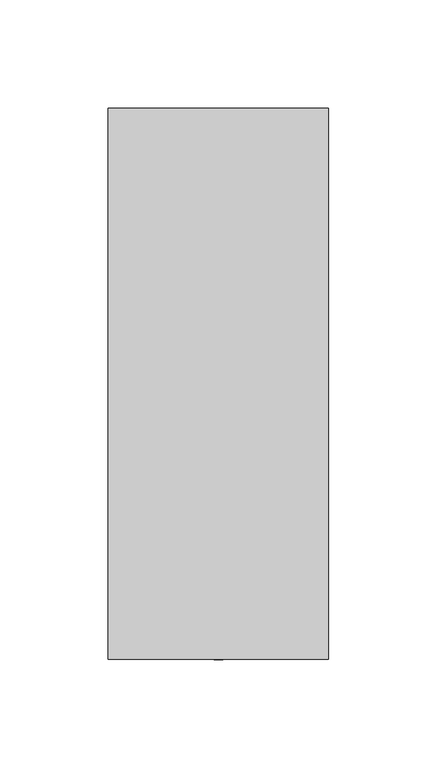
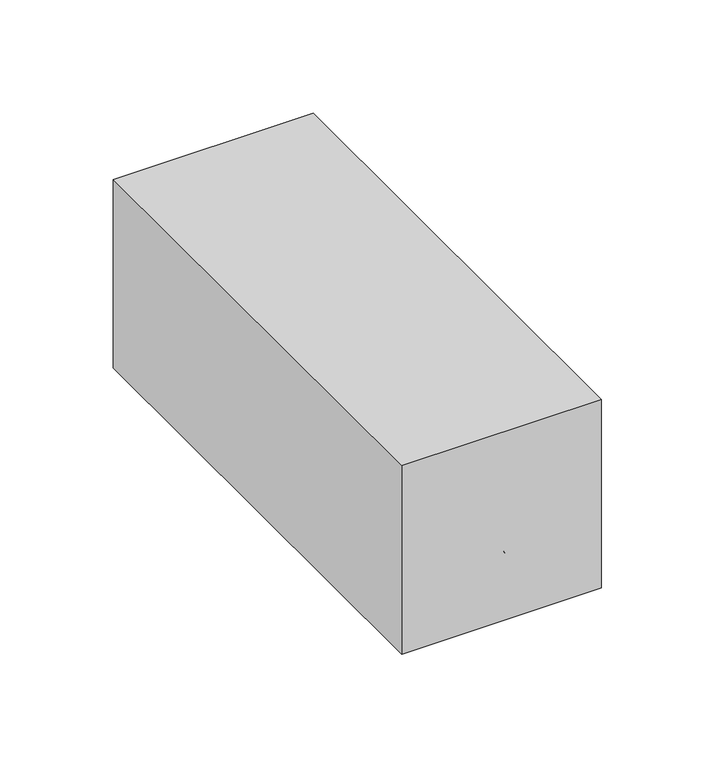
"""IFC4 building model written with IfcOpenShell, lengths in millimetres: proxy geometry, M0750 - Flowmeter, Air, Connect W50 PSI Supply : M0750 - Flowmeter, Air, Connect W50 PSI Supply."""

import ifcopenshell
import ifcopenshell.guid

model = None  # the IFC model being written
_history = None  # IfcOwnerHistory: only IFC2X3 demands one
_inside = {}  # id of a spatial element -> (the spatial element, [elements in it])
_under = {}  # id of a project, library or spatial element -> (it, [spatial elements below it])
_declared = {}  # id of a project -> (the project, [libraries it declares])
_typed = {}  # id of a type object -> (the type object, [elements of that type])
_made_of = {}  # id of a material, layer set ... -> (it, [elements and type objects made of it])


def new_model(schema):
    """Start an empty IFC model of exactly this schema.

    Asked for "IFC4X3", IfcOpenShell would pick the latest addendum, in which some entities
    have other attributes; the version numbers below select the first issue.
    IFC2X3 requires an IfcOwnerHistory on every rooted entity: one is made here for all.
    """
    global model, _history
    if schema == "IFC4X3":
        model = ifcopenshell.file(schema_version=(4, 3, 0, 0))
    else:
        model = ifcopenshell.file(schema=schema)
    _inside.clear()
    _under.clear()
    _declared.clear()
    _typed.clear()
    _made_of.clear()
    _history = None
    if model.schema == "IFC2X3":
        org = make("IfcOrganization", Name="unknown")
        user = make(
            "IfcPersonAndOrganization",
            ThePerson=make("IfcPerson", FamilyName="unknown"),
            TheOrganization=org,
        )
        app = make(
            "IfcApplication",
            ApplicationDeveloper=org,
            Version="unknown",
            ApplicationFullName="unknown",
            ApplicationIdentifier="unknown",
        )
        _history = make(
            "IfcOwnerHistory",
            OwningUser=user,
            OwningApplication=app,
            ChangeAction="ADDED",
            CreationDate=0,
        )
    return model


def make(cls, **values):
    """One entity of the class cls with the attributes given. An attribute that is None is left unset."""
    return model.create_entity(
        cls, **{name: value for name, value in values.items() if value is not None}
    )


def rooted(cls, **values):
    """An entity with a GlobalId (a new one), such as an element, a storey or a relation."""
    return make(cls, GlobalId=ifcopenshell.guid.new(), OwnerHistory=_history, **values)


def si_unit(unit_type, name, prefix=None):
    """IfcSIUnit, for example si_unit("LENGTHUNIT", "METRE", prefix="MILLI")."""
    return make("IfcSIUnit", UnitType=unit_type, Prefix=prefix, Name=name)


def assignment(units):
    """IfcUnitAssignment: the units of a project."""
    return None if units is None else make("IfcUnitAssignment", Units=units)


def point(xyz):
    """IfcCartesianPoint."""
    return None if xyz is None else make("IfcCartesianPoint", Coordinates=xyz)


def direction(xyz):
    """IfcDirection."""
    return None if xyz is None else make("IfcDirection", DirectionRatios=xyz)


def frame(location, z_axis=None, x_axis=None):
    """IfcAxis2Placement3D, a coordinate frame: its origin and axes. An axis left out is left unset."""
    return make(
        "IfcAxis2Placement3D",
        Location=point(location),
        Axis=direction(z_axis),
        RefDirection=direction(x_axis),
    )


def frame_2d(location, x_axis=None):
    """IfcAxis2Placement2D, a coordinate frame in the plane: its origin and x axis."""
    return make(
        "IfcAxis2Placement2D", Location=point(location), RefDirection=direction(x_axis)
    )


def origin():
    """The frame at (0, 0, 0) with its axes left unset."""
    return frame((0.0, 0.0, 0.0))


def origin_with_axes():
    """The frame at (0, 0, 0) with the z axis (0, 0, 1) and the x axis (1, 0, 0) written out."""
    return frame((0.0, 0.0, 0.0), z_axis=(0.0, 0.0, 1.0), x_axis=(1.0, 0.0, 0.0))


def place(relative_to, where):
    """IfcLocalPlacement: puts the frame where relative to a parent placement (None: the world)."""
    return make(
        "IfcLocalPlacement", PlacementRelTo=relative_to, RelativePlacement=where
    )


def context(
    kind, dimensions, precision=None, world=None, true_north=None, identifier=None
):
    """IfcGeometricRepresentationContext, for example the 3D "Model" context."""
    return make(
        "IfcGeometricRepresentationContext",
        ContextIdentifier=identifier,
        ContextType=kind,
        CoordinateSpaceDimension=dimensions,
        Precision=precision,
        WorldCoordinateSystem=world,
        TrueNorth=true_north,
    )


def project(units=None, contexts=None):
    """IfcProject with its units and contexts."""
    return rooted(
        "IfcProject",
        Name="project",
        RepresentationContexts=contexts,
        UnitsInContext=assignment(units),
    )


def spatial(cls, under=None, at=None, **own):
    """A site, building, storey or space (cls), placed at a placement, below another one or the project."""
    s = rooted(cls, ObjectPlacement=at, **own)
    if under is not None:
        _under.setdefault(under.id(), (under, []))[1].append(s)
    return s


def polyline(points):
    """IfcPolyline through the points."""
    return make("IfcPolyline", Points=[point(p) for p in points])


def circle_curve(where, radius):
    """IfcCircle in the frame where."""
    return make("IfcCircle", Position=where, Radius=radius)


def trimmed(basis, trim1, trim2, sense, master):
    """IfcTrimmedCurve: the piece of a basis curve between two trims."""
    return make(
        "IfcTrimmedCurve",
        BasisCurve=basis,
        Trim1=trim1,
        Trim2=trim2,
        SenseAgreement=sense,
        MasterRepresentation=master,
    )


def segment(curve, same_sense, transition):
    """IfcCompositeCurveSegment."""
    return make(
        "IfcCompositeCurveSegment",
        Transition=transition,
        SameSense=same_sense,
        ParentCurve=curve,
    )


def composite_curve(segments, self_intersect=None):
    """IfcCompositeCurve: segments joined end to end."""
    return make("IfcCompositeCurve", Segments=segments, SelfIntersect=self_intersect)


def outline(outer, holes=None, kind="AREA"):
    """IfcArbitraryClosedProfileDef: a profile drawn as a closed curve; with holes, ...WithVoids."""
    if holes is None:
        return make("IfcArbitraryClosedProfileDef", ProfileType=kind, OuterCurve=outer)
    return make(
        "IfcArbitraryProfileDefWithVoids",
        ProfileType=kind,
        OuterCurve=outer,
        InnerCurves=holes,
    )


def extrude(swept, where, along, depth):
    """IfcExtrudedAreaSolid: the profile swept, set in the frame where, extruded along a direction by depth."""
    return make(
        "IfcExtrudedAreaSolid",
        SweptArea=swept,
        Position=where,
        ExtrudedDirection=direction(along),
        Depth=depth,
    )


def shape(context_of_items, identifier, shape_type, items):
    """IfcShapeRepresentation: the items that make up one representation, for example the "Body"."""
    return make(
        "IfcShapeRepresentation",
        ContextOfItems=context_of_items,
        RepresentationIdentifier=identifier,
        RepresentationType=shape_type,
        Items=items,
    )


def source(mapping_origin, context_of_items, identifier, shape_type, items):
    """IfcRepresentationMap: a shape defined once, which mapped items show again and again."""
    return make(
        "IfcRepresentationMap",
        MappingOrigin=mapping_origin,
        MappedRepresentation=shape(context_of_items, identifier, shape_type, items),
    )


def transform(
    local_origin,
    x_axis=None,
    y_axis=None,
    z_axis=None,
    scale=None,
    scale2=None,
    scale3=None,
    uniform=True,
):
    """IfcCartesianTransformationOperator3D, or its non-uniform kind. x_axis, y_axis, z_axis: its Axis1, 2, 3."""
    if uniform:
        return make(
            "IfcCartesianTransformationOperator3D",
            Axis1=direction(x_axis),
            Axis2=direction(y_axis),
            LocalOrigin=point(local_origin),
            Scale=scale,
            Axis3=direction(z_axis),
        )
    return make(
        "IfcCartesianTransformationOperator3DnonUniform",
        Axis1=direction(x_axis),
        Axis2=direction(y_axis),
        LocalOrigin=point(local_origin),
        Scale=scale,
        Axis3=direction(z_axis),
        Scale2=scale2,
        Scale3=scale3,
    )


def mapped(mapping_source, mapping_target):
    """IfcMappedItem: shows the shape of a source again, moved by a transform."""
    return make(
        "IfcMappedItem", MappingSource=mapping_source, MappingTarget=mapping_target
    )


def made_of(thing, what):
    """Note that an element or type object is made of a material, layer set ...; save() writes the relation."""
    if what is not None:
        _made_of.setdefault(what.id(), (what, []))[1].append(thing)
    return thing


def element(
    cls,
    number,
    at=None,
    inside=None,
    cuts=None,
    type_object=None,
    material=None,
    context=None,
    identifier="Body",
    shape_type=None,
    held_by="IfcProductDefinitionShape",
    body=None,
    shapes=None,
    **own,
):
    """One element of the class cls, such as IfcWall. Its Tag is "e" and its number.

    at: its placement. inside: the storey or other place that contains it. cuts: it is an
    opening in that element (IfcRelVoidsElement). A single representation is given by context,
    identifier, shape_type and body (its items); several are given by shapes. held_by: the class
    of the entity that holds the representations. save() writes the other relations.
    """
    e = rooted(cls, Tag="e%d" % number, ObjectPlacement=at, **own)
    if body is not None:
        shapes = [shape(context, identifier, shape_type, body)]
    if shapes is not None:
        e.Representation = make(held_by, Representations=shapes)
    if inside is not None:
        _inside.setdefault(inside.id(), (inside, []))[1].append(e)
    if cuts is not None:
        rooted(
            "IfcRelVoidsElement", RelatingBuildingElement=cuts, RelatedOpeningElement=e
        )
    if type_object is not None:
        _typed.setdefault(type_object.id(), (type_object, []))[1].append(e)
    return made_of(e, material)


def aggregate(whole, parts):
    """IfcRelAggregates: a whole, such as a stair, and the parts it consists of."""
    return rooted("IfcRelAggregates", RelatingObject=whole, RelatedObjects=parts)


def save(model, path):
    """Write the relations noted so far, then the file.

    IfcRelAggregates (storeys below a building ...), IfcRelContainedInSpatialStructure (elements
    in a storey), IfcRelDefinesByType, IfcRelAssociatesMaterial and IfcRelDeclares: one each for
    every whole, place, type object, material and project.
    """
    for whole, parts in _under.values():
        aggregate(whole, parts)
    for where, things in _inside.values():
        rooted(
            "IfcRelContainedInSpatialStructure",
            RelatedElements=things,
            RelatingStructure=where,
        )
    for kind, things in _typed.values():
        rooted("IfcRelDefinesByType", RelatedObjects=things, RelatingType=kind)
    for what, things in _made_of.values():
        rooted("IfcRelAssociatesMaterial", RelatedObjects=things, RelatingMaterial=what)
    for by, libraries in _declared.values():
        rooted("IfcRelDeclares", RelatingContext=by, RelatedDefinitions=libraries)
    model.write(path)


def plane_surface(at):
    """IfcPlane: the flat surface through the origin of the frame at, square to its z axis."""
    return make("IfcPlane", Position=at)


def cylinder_surface(at, radius):
    """IfcCylindricalSurface: all points at the distance radius from the z axis of the frame at."""
    return make("IfcCylindricalSurface", Position=at, Radius=radius)


def revolved_surface(curve, axis_point, axis_direction):
    """IfcSurfaceOfRevolution: the curve turned about the line through axis_point along axis_direction."""
    return make(
        "IfcSurfaceOfRevolution",
        SweptCurve=make("IfcArbitraryOpenProfileDef", ProfileType="CURVE", Curve=curve),
        AxisPosition=make("IfcAxis1Placement", Location=point(axis_point), Axis=direction(axis_direction)),
    )


def advanced_brep(points, edges, surfaces, faces):
    """IfcAdvancedBrep: a solid bounded by faces that lie on surfaces and meet in shared edges.

    An edge is (start, end): straight between two places in points (the first is 0);
    or (start, end, curve); or (start, end, curve, False) where it runs against its curve.
    A face is (place in surfaces, loops), or (place, loops, False) where it looks against
    its surface's normal. A loop lists edges by number (the first is 1), with a minus sign
    where the edge is run from its end to its start. The first loop is the outer one.
    """
    corners = [point(p) for p in points]
    vertices = [make("IfcVertexPoint", VertexGeometry=c) for c in corners]
    made = []
    for start, end, *more in edges:
        made.append(
            make(
                "IfcEdgeCurve",
                EdgeStart=vertices[start],
                EdgeEnd=vertices[end],
                EdgeGeometry=more[0] if more else make("IfcPolyline", Points=[corners[start], corners[end]]),
                SameSense=more[1] if len(more) > 1 else True,
            )
        )
    hull = []
    for where, loops, *sense in faces:
        bounds = []
        for j, loop in enumerate(loops):
            ring = [make("IfcOrientedEdge", EdgeElement=made[abs(k) - 1], Orientation=k > 0) for k in loop]
            bounds.append(
                make(
                    "IfcFaceOuterBound" if j == 0 else "IfcFaceBound",
                    Bound=make("IfcEdgeLoop", EdgeList=ring),
                    Orientation=True,
                )
            )
        hull.append(make("IfcAdvancedFace", Bounds=bounds, FaceSurface=surfaces[where], SameSense=sense[0] if sense else True))
    return make("IfcAdvancedBrep", Outer=make("IfcClosedShell", CfsFaces=hull))


def specialty_equipment_235a6406(model_context):
    return source(origin(), model_context, "Body", "SolidModel", [
        extrude(outline(polyline([(-50.8, 254.0), (50.8, 254.0), (50.8, 0.0), (-50.8, 0.0), (-50.8, 254.0)])), origin_with_axes(), (0.0, 0.0, 1.0), 101.6),
        extrude(outline(composite_curve([segment(trimmed(circle_curve(frame_2d((0.0, 43.7511243)), 11.1125), [point((-11.1125, 43.7511243))], [point((11.1125, 43.7511243))], False, "CARTESIAN"), True, "CONTINUOUS"), segment(trimmed(circle_curve(frame_2d((0.0, 43.7511243)), 11.1125), [point((11.1125, 43.7511243))], [point((-11.1125, 43.7511243))], False, "CARTESIAN"), True, "CONTINUOUS")], self_intersect=False)), origin_with_axes(), (0.0, 0.0, 1.0), 12.1432676),
        extrude(outline(composite_curve([segment(trimmed(circle_curve(frame_2d((0.0, 43.7511243)), 6.35), [point((-6.35, 43.7511243))], [point((6.35, 43.7511243))], False, "CARTESIAN"), True, "CONTINUOUS"), segment(trimmed(circle_curve(frame_2d((0.0, 43.7511243)), 6.35), [point((6.35, 43.7511243))], [point((-6.35, 43.7511243))], False, "CARTESIAN"), True, "CONTINUOUS")], self_intersect=False)), frame((0.0, 0.0, 12.1432676), z_axis=(0.0, 0.0, 1.0), x_axis=(1.0, 0.0, 0.0)), (0.0, 0.0, 1.0), 11.6740858),
        extrude(outline(composite_curve([segment(trimmed(circle_curve(frame_2d((0.0, 43.7511243)), 11.1125), [point((-11.1125, 43.7511243))], [point((11.1125, 43.7511243))], False, "CARTESIAN"), True, "CONTINUOUS"), segment(trimmed(circle_curve(frame_2d((0.0, 43.7511243)), 11.1125), [point((11.1125, 43.7511243))], [point((-11.1125, 43.7511243))], False, "CARTESIAN"), True, "CONTINUOUS")], self_intersect=False)), frame((0.0, 0.0, 12.8429111), z_axis=(0.0, 0.0, 1.0), x_axis=(1.0, 0.0, 0.0)), (0.0, 0.0, 1.0), 3.7345018),
        advanced_brep(
        [(0.0, 195.0035492, 41.6430751), (0.0, 195.0035492, 28.9430751), (0.0, 77.2962509, 43.2305751), (0.0, 77.2962509, 27.3555751)],
        [
            (0, 1, circle_curve(frame((0.0, 195.0035492, 35.2930751), z_axis=(0.0, 1.0, 0.0), x_axis=(0.0, 0.0, 1.0)), 6.35)),
            (1, 0, circle_curve(frame((0.0, 195.0035492, 35.2930751), z_axis=(0.0, 1.0, 0.0), x_axis=(0.0, 0.0, -1.0)), 6.35)),
            (2, 3, circle_curve(frame((0.0, 77.2962509, 35.2930751), z_axis=(0.0, -1.0, 0.0), x_axis=(0.0, 0.0, -1.0)), 7.9375)),
            (3, 2, circle_curve(frame((0.0, 77.2962509, 35.2930751), z_axis=(0.0, -1.0, 0.0), x_axis=(0.0, 0.0, 1.0)), 7.9375)),
            (3, 1),
            (0, 2),
        ],
        [
            plane_surface(frame((0.0, 195.0035492, 35.2930751), z_axis=(0.0, 1.0, 0.0), x_axis=(1.0, 0.0, 0.0))),
            plane_surface(frame((0.0, 77.2962509, 35.2930751), z_axis=(0.0, -1.0, 0.0), x_axis=(1.0, 0.0, 0.0))),
            revolved_surface(polyline([(0.0, 195.0035492, 41.64307510053948), (0.0, 77.29625090000002, 43.2305751)]), (0.0, 665.8327426, 35.2930751), (0.0, -1.0, 0.0)),
            revolved_surface(polyline([(0.0, 195.0035492, 28.943075099460525), (0.0, 77.29625090000002, 27.3555751)]), (0.0, 665.8327426, 35.2930751), (0.0, -1.0, 0.0)),
        ],
        [
            (0, [[1, 2]]),
            (1, [[3, 4]]),
            (2, [[-4, 5, -1, 6]]),
            (3, [[-3, -6, -2, -5]]),
        ],
    ),
        extrude(outline(composite_curve([segment(trimmed(circle_curve(frame_2d((0.0, 56.2938544)), 15.875), [point((-15.875, 56.2938544))], [point((15.875, 56.2938544))], False, "CARTESIAN"), True, "CONTINUOUS"), segment(trimmed(circle_curve(frame_2d((0.0, 56.2938544)), 15.875), [point((15.875, 56.2938544))], [point((-15.875, 56.2938544))], False, "CARTESIAN"), True, "CONTINUOUS")], self_intersect=False)), frame((0.0, 0.0, 73.7139717), z_axis=(0.0, 0.0, 1.0), x_axis=(1.0, 0.0, 0.0)), (0.0, 0.0, 1.0), 9.1021363),
        advanced_brep(
        [(0.0, 197.9462509, 44.8180751), (0.0, 197.9462509, 25.7680751), (0.0, 77.2962509, 46.4055751), (0.0, 77.2962509, 24.1805751)],
        [
            (0, 1, circle_curve(frame((0.0, 197.9462509, 35.2930751), z_axis=(0.0, 1.0, 0.0), x_axis=(0.0, 0.0, 1.0)), 9.525)),
            (1, 0, circle_curve(frame((0.0, 197.9462509, 35.2930751), z_axis=(0.0, 1.0, 0.0), x_axis=(0.0, 0.0, -1.0)), 9.525)),
            (2, 3, circle_curve(frame((0.0, 77.2962509, 35.2930751), z_axis=(0.0, -1.0, 0.0), x_axis=(0.0, 0.0, -1.0)), 11.1125)),
            (3, 2, circle_curve(frame((0.0, 77.2962509, 35.2930751), z_axis=(0.0, -1.0, 0.0), x_axis=(0.0, 0.0, 1.0)), 11.1125)),
            (3, 1),
            (0, 2),
        ],
        [
            plane_surface(frame((0.0, 197.9462509, 35.2930751), z_axis=(0.0, 1.0, 0.0), x_axis=(1.0, 0.0, 0.0))),
            plane_surface(frame((0.0, 77.2962509, 35.2930751), z_axis=(0.0, -1.0, 0.0), x_axis=(1.0, 0.0, 0.0))),
            revolved_surface(polyline([(0.0, 197.9462509, 44.8180751), (0.0, 77.29625090000002, 46.4055751)]), (0.0, 921.8462509, 35.2930751), (0.0, -1.0, 0.0)),
            revolved_surface(polyline([(0.0, 197.9462509, 25.768075099999997), (0.0, 77.29625090000002, 24.1805751)]), (0.0, 921.8462509, 35.2930751), (0.0, -1.0, 0.0)),
        ],
        [
            (0, [[1, 2]]),
            (1, [[3, 4]]),
            (2, [[-4, 5, -1, 6]]),
            (3, [[-3, -6, -2, -5]]),
        ],
    ),
        advanced_brep(
        [(16.4405012, 77.2962509, 35.2930751), (-16.4405012, 77.2962509, 35.2930751), (0.0, 77.2962509, 35.2930751), (17.4336479, 76.3031042, 35.2930751), (-17.4336479, 76.3031042, 35.2930751), (17.4336479, 64.5962509, 35.2930751), (-17.4336479, 64.5962509, 35.2930751), (14.6960919, 64.5962509, 35.2930751), (-14.6960919, 64.5962509, 35.2930751), (14.6960919, 63.5321613, 35.2930751), (-14.6960919, 63.5321613, 35.2930751), (15.9348033, 63.5321613, 35.2930751), (-15.9348033, 63.5321613, 35.2930751), (15.9348033, 33.3696613, 35.2930751), (-15.9348033, 33.3696613, 35.2930751), (8.893951, 30.7772209, 35.2930751), (-8.893951, 30.7772209, 35.2930751), (4.4469755, 30.7772209, 35.2930751), (-4.4469755, 30.7772209, 35.2930751), (4.4469755, 25.4, 35.2930751), (-4.4469755, 25.4, 35.2930751), (0.0, 25.4, 35.2930751)],
        [
            (0, 1, circle_curve(frame((0.0, 77.2962509, 35.2930751), z_axis=(0.0, 1.0, 0.0), x_axis=(-1.0, 0.0, 0.0)), 16.4405012)),
            (1, 2),
            (2, 0),
            (1, 0, circle_curve(frame((0.0, 77.2962509, 35.2930751), z_axis=(0.0, 1.0, 0.0), x_axis=(-1.0, 0.0, 0.0)), 16.4405012)),
            (3, 4, circle_curve(frame((0.0, 76.3031042, 35.2930751), z_axis=(0.0, 1.0, 0.0), x_axis=(-1.0, 0.0, 0.0)), 17.4336479)),
            (4, 1),
            (0, 3),
            (4, 3, circle_curve(frame((0.0, 76.3031042, 35.2930751), z_axis=(0.0, 1.0, 0.0), x_axis=(-1.0, 0.0, 0.0)), 17.4336479)),
            (5, 6, circle_curve(frame((0.0, 64.5962509, 35.2930751), z_axis=(0.0, 1.0, 0.0), x_axis=(-1.0, 0.0, 0.0)), 17.4336479)),
            (6, 4),
            (3, 5),
            (6, 5, circle_curve(frame((0.0, 64.5962509, 35.2930751), z_axis=(0.0, 1.0, 0.0), x_axis=(-1.0, 0.0, 0.0)), 17.4336479)),
            (7, 8, circle_curve(frame((0.0, 64.5962509, 35.2930751), z_axis=(0.0, 1.0, 0.0), x_axis=(-1.0, 0.0, 0.0)), 14.6960919)),
            (8, 6),
            (5, 7),
            (8, 7, circle_curve(frame((0.0, 64.5962509, 35.2930751), z_axis=(0.0, 1.0, 0.0), x_axis=(-1.0, 0.0, 0.0)), 14.6960919)),
            (9, 10, circle_curve(frame((0.0, 63.5321613, 35.2930751), z_axis=(0.0, 1.0, 0.0), x_axis=(-1.0, 0.0, 0.0)), 14.6960919)),
            (10, 8),
            (7, 9),
            (10, 9, circle_curve(frame((0.0, 63.5321613, 35.2930751), z_axis=(0.0, 1.0, 0.0), x_axis=(-1.0, 0.0, 0.0)), 14.6960919)),
            (11, 12, circle_curve(frame((0.0, 63.5321613, 35.2930751), z_axis=(0.0, 1.0, 0.0), x_axis=(-1.0, 0.0, 0.0)), 15.9348033)),
            (12, 10),
            (9, 11),
            (12, 11, circle_curve(frame((0.0, 63.5321613, 35.2930751), z_axis=(0.0, 1.0, 0.0), x_axis=(-1.0, 0.0, 0.0)), 15.9348033)),
            (13, 14, circle_curve(frame((0.0, 33.3696613, 35.2930751), z_axis=(0.0, 1.0, 0.0), x_axis=(-1.0, 0.0, 0.0)), 15.9348033)),
            (14, 12),
            (11, 13),
            (14, 13, circle_curve(frame((0.0, 33.3696613, 35.2930751), z_axis=(0.0, 1.0, 0.0), x_axis=(-1.0, 0.0, 0.0)), 15.9348033)),
            (15, 16, circle_curve(frame((0.0, 30.7772209, 35.2930751), z_axis=(0.0, 1.0, 0.0), x_axis=(-1.0, 0.0, 0.0)), 8.893951)),
            (16, 14),
            (13, 15),
            (16, 15, circle_curve(frame((0.0, 30.7772209, 35.2930751), z_axis=(0.0, 1.0, 0.0), x_axis=(-1.0, 0.0, 0.0)), 8.893951)),
            (17, 18, circle_curve(frame((0.0, 30.7772209, 35.2930751), z_axis=(0.0, 1.0, 0.0), x_axis=(-1.0, 0.0, 0.0)), 4.4469755)),
            (18, 16),
            (15, 17),
            (18, 17, circle_curve(frame((0.0, 30.7772209, 35.2930751), z_axis=(0.0, 1.0, 0.0), x_axis=(-1.0, 0.0, 0.0)), 4.4469755)),
            (19, 20, circle_curve(frame((0.0, 25.4, 35.2930751), z_axis=(0.0, 1.0, 0.0), x_axis=(-1.0, 0.0, 0.0)), 4.4469755)),
            (20, 18),
            (17, 19),
            (20, 19, circle_curve(frame((0.0, 25.4, 35.2930751), z_axis=(0.0, 1.0, 0.0), x_axis=(-1.0, 0.0, 0.0)), 4.4469755)),
            (21, 20),
            (19, 21),
        ],
        [
            plane_surface(frame((0.0, 77.2962509, 35.2930751), z_axis=(0.0, 1.0, 0.0), x_axis=(-1.0, 0.0, 0.0))),
            revolved_surface(polyline([(-16.4405012, 77.2962509, 35.2930751), (-17.4336479, 76.3031042, 35.2930751)]), (0.0, 77.2962509, 35.2930751), (0.0, -1.0, 0.0)),
            cylinder_surface(frame((0.0, 77.2962509, 35.2930751), z_axis=(0.0, -1.0, 0.0), x_axis=(-1.0, 0.0, 0.0)), 17.4336479),
            plane_surface(frame((0.0, 64.5962509, 35.2930751), z_axis=(0.0, -1.0, 0.0), x_axis=(-1.0, 0.0, 0.0))),
            cylinder_surface(frame((0.0, 77.2962509, 35.2930751), z_axis=(0.0, -1.0, 0.0), x_axis=(-1.0, 0.0, 0.0)), 14.6960919),
            plane_surface(frame((0.0, 63.5321613, 35.2930751), z_axis=(0.0, 1.0, 0.0), x_axis=(-1.0, 0.0, 0.0))),
            cylinder_surface(frame((0.0, 77.2962509, 35.2930751), z_axis=(0.0, -1.0, 0.0), x_axis=(-1.0, 0.0, 0.0)), 15.9348033),
            revolved_surface(polyline([(-15.9348033, 33.3696613, 35.2930751), (-8.893951, 30.7772209, 35.2930751)]), (0.0, 77.2962509, 35.2930751), (0.0, -1.0, 0.0)),
            plane_surface(frame((0.0, 30.7772209, 35.2930751), z_axis=(0.0, -1.0, 0.0), x_axis=(-1.0, 0.0, 0.0))),
            cylinder_surface(frame((0.0, 77.2962509, 35.2930751), z_axis=(0.0, -1.0, 0.0), x_axis=(-1.0, 0.0, 0.0)), 4.4469755),
            plane_surface(frame((0.0, 25.4, 35.2930751), z_axis=(0.0, -1.0, 0.0), x_axis=(-1.0, 0.0, 0.0))),
        ],
        [
            (0, [[1, 2, 3]]),
            (0, [[4, -3, -2]]),
            (1, [[5, 6, -1, 7]]),
            (1, [[8, -7, -4, -6]]),
            (2, [[9, 10, -5, 11]]),
            (2, [[12, -11, -8, -10]]),
            (3, [[13, 14, -9, 15]]),
            (3, [[16, -15, -12, -14]]),
            (4, [[17, 18, -13, 19]]),
            (4, [[20, -19, -16, -18]]),
            (5, [[21, 22, -17, 23]]),
            (5, [[24, -23, -20, -22]]),
            (6, [[25, 26, -21, 27]]),
            (6, [[28, -27, -24, -26]]),
            (7, [[29, 30, -25, 31]]),
            (7, [[32, -31, -28, -30]]),
            (8, [[33, 34, -29, 35]]),
            (8, [[36, -35, -32, -34]]),
            (9, [[37, 38, -33, 39]]),
            (9, [[40, -39, -36, -38]]),
            (10, [[41, -37, 42]]),
            (10, [[-42, -40, -41]]),
        ],
    ),
        extrude(outline(composite_curve([segment(trimmed(circle_curve(frame_2d((0.0, 56.2938544)), 4.7625), [point((-4.7625, 56.2938544))], [point((4.7625, 56.2938544))], False, "CARTESIAN"), True, "CONTINUOUS"), segment(trimmed(circle_curve(frame_2d((0.0, 56.2938544)), 4.7625), [point((4.7625, 56.2938544))], [point((-4.7625, 56.2938544))], False, "CARTESIAN"), True, "CONTINUOUS")], self_intersect=False)), frame((0.0, 0.0, 50.024421), z_axis=(0.0, 0.0, 1.0), x_axis=(1.0, 0.0, 0.0)), (0.0, 0.0, 1.0), 33.6662415),
        extrude(outline(polyline([(-4.0213654, 63.2590636), (4.0213654, 63.2590636), (8.0427308, 56.2938544), (4.0213654, 49.3286452), (-4.0213654, 49.3286452), (-8.0427308, 56.2938544), (-4.0213654, 63.2590636)])), frame((0.0, 0.0, 54.0167391), z_axis=(0.0, 0.0, 1.0), x_axis=(1.0, 0.0, 0.0)), (0.0, 0.0, 1.0), 12.0291395),
        advanced_brep(
        [(5.8611698, 21.8455296, 35.2930751), (-5.8611698, 21.8455296, 35.2930751), (-5.8611698, 25.4, 35.2930751), (5.8611698, 25.4, 35.2930751), (2.0092135, 0.0, 35.2930751), (-2.0092135, 0.0, 35.2930751), (0.0, 0.0, 35.2930751), (0.0, 25.4, 35.2930751)],
        [
            (0, 1, circle_curve(frame((0.0, 21.8455296, 35.2930751), z_axis=(0.0, 1.0, 0.0), x_axis=(-1.0, 0.0, 0.0)), 5.8611698)),
            (1, 2),
            (2, 3, circle_curve(frame((0.0, 25.4, 35.2930751), z_axis=(0.0, -1.0, 0.0), x_axis=(-1.0, 0.0, 0.0)), 5.8611698)),
            (3, 0),
            (1, 0, circle_curve(frame((0.0, 21.8455296, 35.2930751), z_axis=(0.0, 1.0, 0.0), x_axis=(-1.0, 0.0, 0.0)), 5.8611698)),
            (3, 2, circle_curve(frame((0.0, 25.4, 35.2930751), z_axis=(0.0, -1.0, 0.0), x_axis=(-1.0, 0.0, 0.0)), 5.8611698)),
            (4, 5, circle_curve(frame((0.0, 0.0, 35.2930751), z_axis=(0.0, 1.0, 0.0), x_axis=(-1.0, 0.0, 0.0)), 2.0092135)),
            (5, 1),
            (0, 4),
            (5, 4, circle_curve(frame((0.0, 0.0, 35.2930751), z_axis=(0.0, 1.0, 0.0), x_axis=(-1.0, 0.0, 0.0)), 2.0092135)),
            (6, 5),
            (4, 6),
            (2, 7),
            (7, 3),
        ],
        [
            cylinder_surface(frame((0.0, 23.4018459, 35.2930751), z_axis=(0.0, -1.0, 0.0), x_axis=(-1.0, 0.0, 0.0)), 5.8611698),
            revolved_surface(polyline([(-5.8611698, 21.8455296, 35.2930751), (-2.0092135, 0.0, 35.2930751)]), (0.0, 23.4018459, 35.2930751), (0.0, -1.0, 0.0)),
            plane_surface(frame((0.0, 0.0, 35.2930751), z_axis=(0.0, -1.0, 0.0), x_axis=(-1.0, 0.0, 0.0))),
            plane_surface(frame((0.0, 25.4, 35.2930751), z_axis=(0.0, 1.0, 0.0), x_axis=(-1.0, 0.0, 0.0))),
        ],
        [
            (0, [[1, 2, 3, 4]]),
            (0, [[5, -4, 6, -2]]),
            (1, [[7, 8, -1, 9]]),
            (1, [[10, -9, -5, -8]]),
            (2, [[11, -7, 12]]),
            (2, [[-12, -10, -11]]),
            (3, [[-3, 13, 14]]),
            (3, [[-6, -14, -13]]),
        ],
    ),
    ])


if __name__ == "__main__":
    model = new_model("IFC4")
    model_context = context("Model", 3, world=origin())
    ifc_project = project(units=[si_unit("LENGTHUNIT", "METRE", prefix="MILLI")], contexts=[model_context])
    site = spatial("IfcSite", under=ifc_project)
    building = spatial("IfcBuilding", under=site)
    placement = place(None, origin())
    specialty_equipment_shape = specialty_equipment_235a6406(model_context)
    element("IfcBuildingElementProxy", 1, Name="M0750 - Flowmeter, Air, Connect W50 PSI Supply : M0750 - Flowmeter, Air, Connect W50 PSI Supply", ObjectType="M0750 - Flowmeter, Air, Connect W50 PSI Supply : M0750 - Flowmeter, Air, Connect W50 PSI Supply", at=placement, inside=building, context=model_context, shape_type="MappedRepresentation", body=[
        mapped(specialty_equipment_shape, transform((0.0, 0.0, 0.0), x_axis=(1.0, 0.0, 0.0), y_axis=(0.0, 1.0, 0.0), z_axis=(0.0, 0.0, 1.0))),
    ])
    save(model, "model.ifc")

# Revit data of these elements
# Type "M0750 - Flowmeter, Air, Connect W50 PSI Supply : M0750 - Flowmeter, Air, Connect W50 PSI Supply"
#   Watts2 = "0"
#   Watts1 = "0"
#   Unit_Issue = "EA"
#   UTIL_6_Misc = "-"
#   UTIL_5_NonMedGas = "-"
#   UTIL_4_MiscGas = "-"
#   UTIL_3_MedGas = "K"
#   UTIL_2_Elec = "-"
#   UTIL_1_WaterDrain = "-"
#   Nomenclature = "Flowmeter, Air, Connect w/50 PSI Supply"
#   NSN = "6530"
#   Location [instance default] = ""
#   JSN = "M0750"
#   Fund_Source_VA = "-"
#   Fund_Source_Navy = "-"
#   Fund_Source_Army = "-"
#   Fund_Source_AF = "-"
#   ELEC_Volts2 = "0"
#   ELEC_Volts1 = "0"
#   ELEC_Phase2 = "0"
#   ELEC_Phase1 = "0"
#   ELEC_HertzSwitch = "0"
#   ELEC_HertzDependent = "0"
#   ELEC_Hertz = "0"
#   ELEC_Amps2 = "0"
#   ELEC_Amps1 = "0"
#   DetailDescription = "Air flowmeter. Unit has a stainless steel needle valve with clear flowtube for connection to 50 PSI air outlet from central pipeline system. Requires the appropriate adapter for connection to the wall outlet and fitting to connect to tubing. Database prices reflect fittings with an attached DISS power outlet. Other outlet and adapter configurations are available."
#   CAT_VA = "C"
#   CAT_Navy = "C"
#   CAT_IHS = "-"
#   CAT_Army = "C"
#   CAT_AF = "C"
#   BTUperhour = "0"
#   Weight_IP = 3
#   Default Elevation = 4' - 0"
#   DIM_Width_IP = 0' - 4"
#   DIM_Height_IP = 0' - 10"
#   DIM_Depth_IP = 0' - 4"
#   finish [instance default] = none
# Element 1 (IfcBuildingElementProxy, "M0750 - Flowmeter, Air, Connect W50 PSI Supply : M0750 - Flowmeter, Air, Connect W50 PSI Supply")
#   Location = "BRMS1"
#   Materials on its faces: "Glass", "EquipSpace"
# Materials
#   "Glass": class "Glass", colour RGB 0 128 192, transparency 0.75
#   "EquipSpace": class "Unassigned", colour RGB 221 217 195, transparency 0.5
